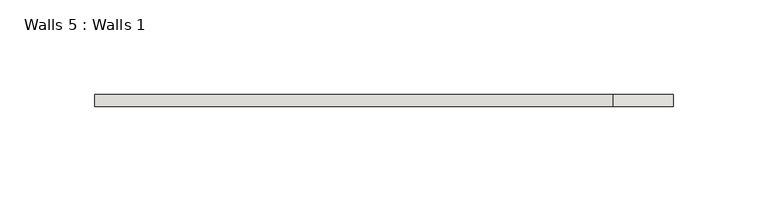
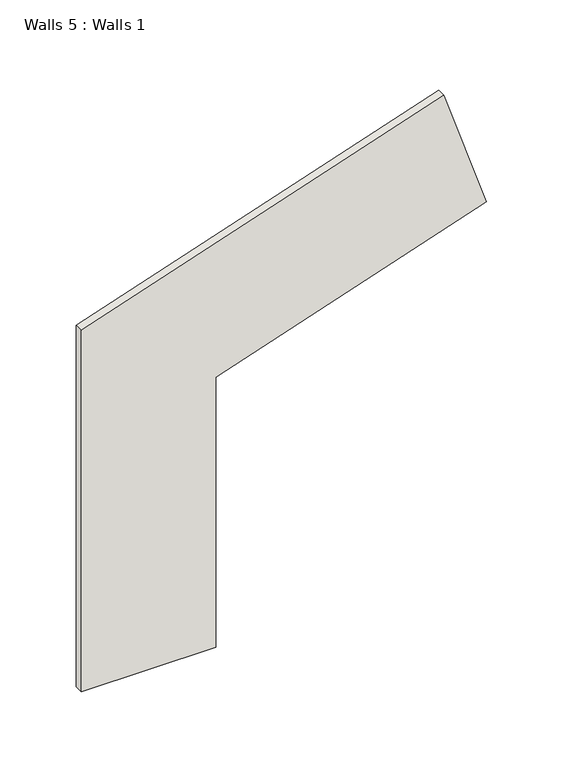
"""IFC4 building model written with IfcOpenShell, lengths in millimetres: wall geometry, Walls 5 : Walls 1."""

from ifc_helpers import new_model, si_unit, frame, origin, place, context, project, spatial, polyline, outline, extrude, source, transform, mapped, element, save


def walls_5_walls_1_e7ce3408(model_context):
    return source(origin(), model_context, "Body", "SweptSolid", [
        extrude(outline(polyline([(5071.1413299, 19768.3370052), (4782.1134335, 19768.3370052), (4782.1134335, 19869.9370052), (4998.0134335, 19869.9370052), (5066.5557127, 20074.6679651), (5162.8996939, 20042.4127749), (5071.1413299, 19768.3370052)])), frame((0.0, -976.6384634, 0.0), z_axis=(0.0, 1.0, 0.0), x_axis=(0.0, 0.0, 1.0)), (0.0, 0.0, 1.0), 6.35),
    ])


if __name__ == "__main__":
    model = new_model("IFC4")
    model_context = context("Model", 3, world=origin())
    ifc_project = project(units=[si_unit("LENGTHUNIT", "METRE", prefix="MILLI")], contexts=[model_context])
    site = spatial("IfcSite", under=ifc_project)
    building = spatial("IfcBuilding", under=site)
    placement = place(None, origin())
    walls_5_walls_1_shape = walls_5_walls_1_e7ce3408(model_context)
    element("IfcWall", 1, ObjectType="Walls 5 : Walls 1", at=placement, inside=building, context=model_context, shape_type="MappedRepresentation", body=[
        mapped(walls_5_walls_1_shape, transform((0.0, 0.0, 0.0), x_axis=(1.0, 0.0, 0.0), y_axis=(0.0, 1.0, 0.0), z_axis=(0.0, 0.0, 1.0))),
    ])
    save(model, "model.ifc")

# Revit data of these elements
# Element 1 (IfcWall, "Walls 5 : Walls 1")
#   Materials on its faces: "1/4\" STEEL GUSSET PLATE - (RAW STEEL)"
# Materials
#   "1/4\" STEEL GUSSET PLATE - (RAW STEEL)": class "Metal", colour RGB 189 187 185, transparency 0, Description = "Structural steel 50ksi", Cost = 0
